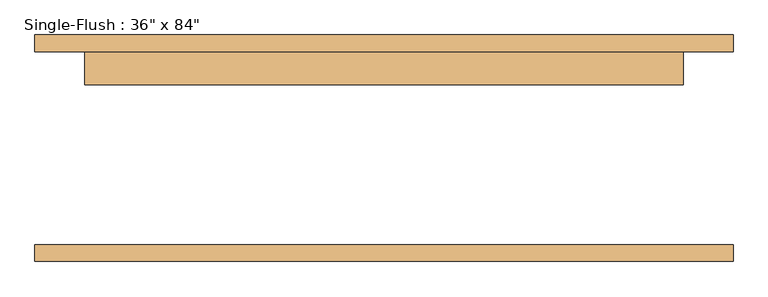
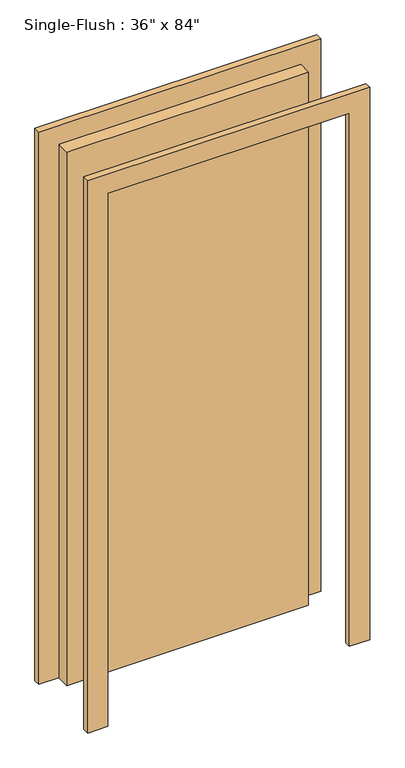
"""IFC4 building model written with IfcOpenShell, lengths in millimetres: door geometry."""

from ifc_helpers import new_model, si_unit, frame, origin, origin_with_axes, place, context, project, spatial, polyline, outline, extrude, source, transform, mapped, element, save


def door_7b231ec9(model_context):
    return source(origin(), model_context, "Body", "SweptSolid", [
        extrude(outline(polyline([(2209.8, -533.4), (0.0, -533.4), (0.0, -457.2), (2133.6, -457.2), (2133.6, 457.2), (0.0, 457.2), (0.0, 533.4), (2209.8, 533.4), (2209.8, -533.4)])), frame((0.0, 147.6375, 0.0), z_axis=(0.0, 1.0, 0.0), x_axis=(0.0, 0.0, 1.0)), (0.0, 0.0, 1.0), 25.4),
        extrude(outline(polyline([(2209.8, 533.4), (2209.8, -533.4), (0.0, -533.4), (0.0, -457.2), (2133.6, -457.2), (2133.6, 457.2), (0.0, 457.2), (0.0, 533.4), (2209.8, 533.4)])), frame((0.0, -173.0375, 0.0), z_axis=(0.0, 1.0, 0.0), x_axis=(0.0, 0.0, 1.0)), (0.0, 0.0, 1.0), 25.4),
        extrude(outline(polyline([(457.2, 96.8375), (-457.2, 96.8375), (-457.2, 147.6375), (457.2, 147.6375), (457.2, 96.8375)])), origin_with_axes(), (0.0, 0.0, 1.0), 2133.6),
    ])


if __name__ == "__main__":
    model = new_model("IFC4")
    model_context = context("Model", 3, world=origin())
    ifc_project = project(units=[si_unit("LENGTHUNIT", "METRE", prefix="MILLI")], contexts=[model_context])
    site = spatial("IfcSite", under=ifc_project)
    building = spatial("IfcBuilding", under=site)
    placement = place(None, origin())
    door_shape = door_7b231ec9(model_context)
    element("IfcDoor", 1, ObjectType="Single-Flush : 36\" x 84\"", at=placement, inside=building, context=model_context, shape_type="MappedRepresentation", body=[
        mapped(door_shape, transform((0.0, 0.0, 0.0), x_axis=(1.0, 0.0, 0.0), y_axis=(0.0, 1.0, 0.0), z_axis=(0.0, 0.0, 1.0))),
    ])
    save(model, "model.ifc")

# Revit data of these elements
# Type "Single-Flush : 36\" x 84\""
#   Type Mark = "1"
#   Construction Type Id = "MDOOR"
#   Assembly Code = "C1020"
#   Analytic Construction = "Metal"
#   Thickness = 0' - 2"
#   Heat Transfer Coefficient (U) = 0.651978 BTU/(h·ft²·°F)
#   Height = 7' - 0"
#   Trim Projection Ext = 0' - 1"
#   Trim Projection Int = 0' - 1"
#   Trim Width = 0' - 3"
#   Width = 3' - 0"
#   Define Thermal Properties by = 1
#   Define Thermal Properties by = 1
#   Door Material = Door - Panel
#   Frame Material = Door - Frame
#   Visual Light Transmittance = 0
#   Solar Heat Gain Coefficient = 0
#   Function = (empty or 0)
#   Wall Closure = (empty or 0)
# Element 1 (IfcDoor, "Single-Flush : 36\" x 84\"")
#   Materials on its faces: "Door - Frame", "Door - Panel"
# Materials
#   "Door - Panel": class "Wood", colour RGB 210 159 95, transparency 0, Cost = 0
#   "Door - Frame": class "Miscellaneous", colour RGB 118 70 51, transparency 0, Cost = 0
